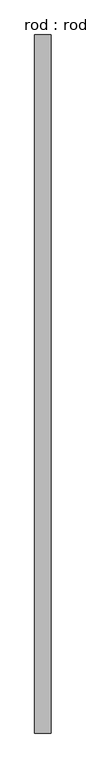
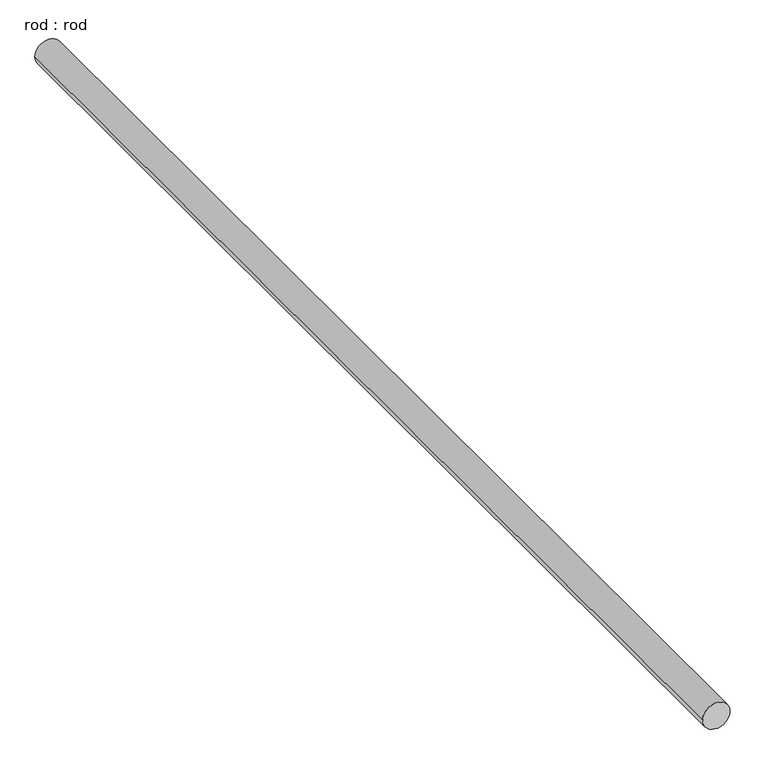
"""IFC4 building model written with IfcOpenShell, lengths in millimetres: proxy geometry, rod : rod."""

from ifc_helpers import new_model, si_unit, point, frame, frame_2d, origin, place, context, project, spatial, circle_curve, trimmed, segment, composite_curve, outline, extrude, source, transform, mapped, element, save


def rod_rod_88b0855c(model_context):
    return source(origin(), model_context, "Body", "SweptSolid", [
        extrude(outline(composite_curve([segment(trimmed(circle_curve(frame_2d((0.0108462, 0.0)), 200.0), [point((0.0108462, 200.0))], [point((0.0108462, -200.0))], False, "CARTESIAN"), True, "CONTINUOUS"), segment(trimmed(circle_curve(frame_2d((0.0108462, 0.0)), 200.0), [point((0.0108462, -200.0))], [point((0.0108462, 200.0))], False, "CARTESIAN"), True, "CONTINUOUS")], self_intersect=False)), frame((0.0, -4395.3251221, 0.0), z_axis=(0.0, 1.0, 0.0), x_axis=(0.0, 0.0, 1.0)), (0.0, 0.0, 1.0), 16976.1074749),
    ])


if __name__ == "__main__":
    model = new_model("IFC4")
    model_context = context("Model", 3, world=origin())
    ifc_project = project(units=[si_unit("LENGTHUNIT", "METRE", prefix="MILLI")], contexts=[model_context])
    site = spatial("IfcSite", under=ifc_project)
    building = spatial("IfcBuilding", under=site)
    placement = place(None, origin())
    rod_rod_shape = rod_rod_88b0855c(model_context)
    element("IfcBuildingElementProxy", 1, Name="rod : rod", ObjectType="rod : rod", at=placement, inside=building, context=model_context, shape_type="MappedRepresentation", body=[
        mapped(rod_rod_shape, transform((0.0, 0.0, 0.0), x_axis=(1.0, 0.0, 0.0), y_axis=(0.0, 1.0, 0.0), z_axis=(0.0, 0.0, 1.0))),
    ])
    save(model, "model.ifc")

# Revit data of these elements
# Type "rod : rod"
#   Default Elevation = 0
